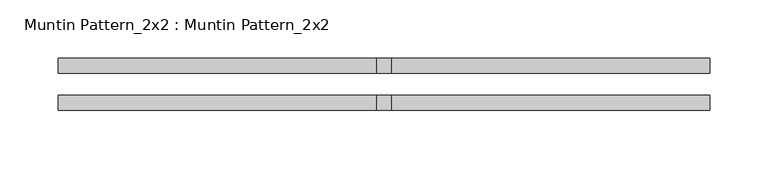
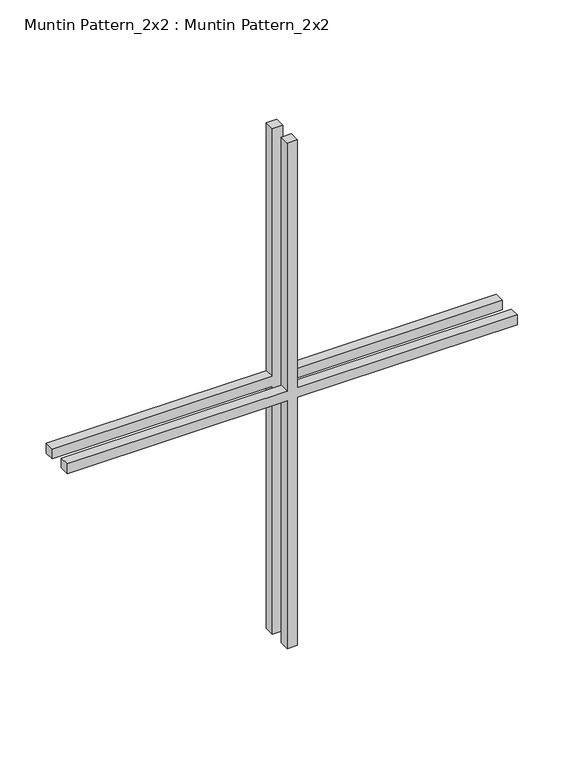
"""IFC4 building model written with IfcOpenShell, lengths in millimetres: proxy geometry, Muntin Pattern_2x2 : Muntin Pattern_2x2."""

from ifc_helpers import new_model, si_unit, frame, origin, place, context, project, spatial, polyline, outline, extrude, source, transform, mapped, element, save


def muntin_pattern_2x2_muntin_pattern_2x2_08c26335(model_context):
    return source(origin(), model_context, "Body", "SweptSolid", [
        extrude(outline(polyline([(338.1375, -6.35), (338.1375, -279.4), (325.4375, -279.4), (325.4375, -6.35), (0.0, -6.35), (0.0, 6.35), (325.4375, 6.35), (325.4375, 279.4), (338.1375, 279.4), (338.1375, 6.35), (663.575, 6.35), (663.575, -6.35), (338.1375, -6.35)])), frame((0.0, 9.525, 0.0), z_axis=(0.0, 1.0, 0.0), x_axis=(0.0, 0.0, 1.0)), (0.0, 0.0, 1.0), 12.7),
        extrude(outline(polyline([(338.1375, -6.35), (338.1375, -279.4), (325.4375, -279.4), (325.4375, -6.35), (0.0, -6.35), (0.0, 6.35), (325.4375, 6.35), (325.4375, 279.4), (338.1375, 279.4), (338.1375, 6.35), (663.575, 6.35), (663.575, -6.35), (338.1375, -6.35)])), frame((0.0, -22.225, 0.0), z_axis=(0.0, 1.0, 0.0), x_axis=(0.0, 0.0, 1.0)), (0.0, 0.0, 1.0), 12.7),
    ])


if __name__ == "__main__":
    model = new_model("IFC4")
    model_context = context("Model", 3, world=origin())
    ifc_project = project(units=[si_unit("LENGTHUNIT", "METRE", prefix="MILLI")], contexts=[model_context])
    site = spatial("IfcSite", under=ifc_project)
    building = spatial("IfcBuilding", under=site)
    placement = place(None, origin())
    muntin_pattern_2x2_muntin_pattern_2x2_shape = muntin_pattern_2x2_muntin_pattern_2x2_08c26335(model_context)
    element("IfcBuildingElementProxy", 1, Name="Muntin Pattern_2x2 : Muntin Pattern_2x2", ObjectType="Muntin Pattern_2x2 : Muntin Pattern_2x2", at=placement, inside=building, context=model_context, shape_type="MappedRepresentation", body=[
        mapped(muntin_pattern_2x2_muntin_pattern_2x2_shape, transform((0.0, 0.0, 0.0), x_axis=(1.0, 0.0, 0.0), y_axis=(0.0, 1.0, 0.0), z_axis=(0.0, 0.0, 1.0))),
    ])
    save(model, "model.ifc")

# Revit data of these elements
# Type "Muntin Pattern_2x2 : Muntin Pattern_2x2"
#   Width [instance default] = 4' - 0"
#   Thickness = 0' - 0 1/2"
#   Height [instance default] = 4' - 0"
#   Distance = 0' - 0 3/4"
#   Interior Material [instance default] = none
#   Exterior Material [instance default] = none
#   Default Elevation = 0
# Element 1 (IfcBuildingElementProxy, "Muntin Pattern_2x2 : Muntin Pattern_2x2")
#   Width = 1' - 10"
#   Height = 2' - 2 1/8"
#   Interior Material = Wood - Stained
#   Exterior Material = Clad - White
#   Materials on its faces: "Clad - White", "Wood - Stained"
# Materials
#   "Clad - White": class "Wood", colour RGB 242 242 238, transparency 0, Cost = 0
#   "Wood - Stained": class "Wood", colour RGB 224 178 126, transparency 0, Cost = 0
